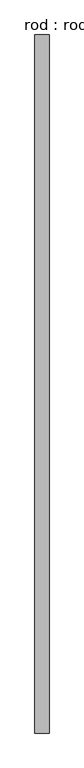
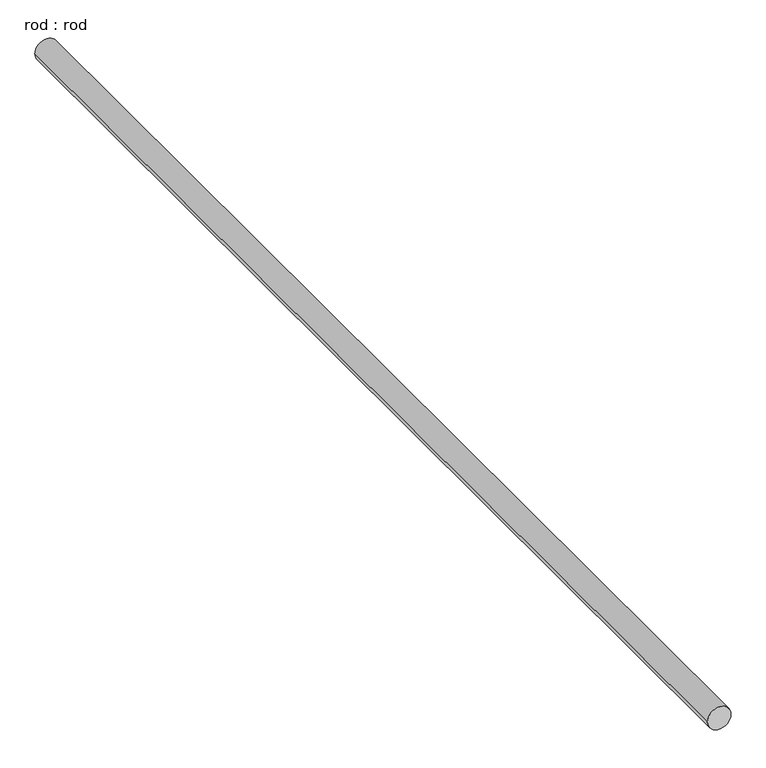
"""IFC4 building model written with IfcOpenShell, lengths in millimetres: proxy geometry, rod : rod."""

from ifc_helpers import new_model, si_unit, point, frame, frame_2d, origin, place, context, project, spatial, circle_curve, trimmed, segment, composite_curve, outline, extrude, source, transform, mapped, element, save


def rod_rod_ac269977(model_context):
    return source(origin(), model_context, "Body", "SweptSolid", [
        extrude(outline(composite_curve([segment(trimmed(circle_curve(frame_2d((0.0108462, 0.0)), 200.0), [point((0.0108462, 200.0))], [point((0.0108462, -200.0))], False, "CARTESIAN"), True, "CONTINUOUS"), segment(trimmed(circle_curve(frame_2d((0.0108462, 0.0)), 200.0), [point((0.0108462, -200.0))], [point((0.0108462, 200.0))], False, "CARTESIAN"), True, "CONTINUOUS")], self_intersect=False)), frame((0.0, -5805.2326054, 0.0), z_axis=(0.0, 1.0, 0.0), x_axis=(0.0, 0.0, 1.0)), (0.0, 0.0, 1.0), 19795.9224416),
    ])


if __name__ == "__main__":
    model = new_model("IFC4")
    model_context = context("Model", 3, world=origin())
    ifc_project = project(units=[si_unit("LENGTHUNIT", "METRE", prefix="MILLI")], contexts=[model_context])
    site = spatial("IfcSite", under=ifc_project)
    building = spatial("IfcBuilding", under=site)
    placement = place(None, origin())
    rod_rod_shape = rod_rod_ac269977(model_context)
    element("IfcBuildingElementProxy", 1, Name="rod : rod", ObjectType="rod : rod", at=placement, inside=building, context=model_context, shape_type="MappedRepresentation", body=[
        mapped(rod_rod_shape, transform((0.0, 0.0, 0.0), x_axis=(1.0, 0.0, 0.0), y_axis=(0.0, 1.0, 0.0), z_axis=(0.0, 0.0, 1.0))),
    ])
    save(model, "model.ifc")

# Revit data of these elements
# Type "rod : rod"
#   Default Elevation = 0
